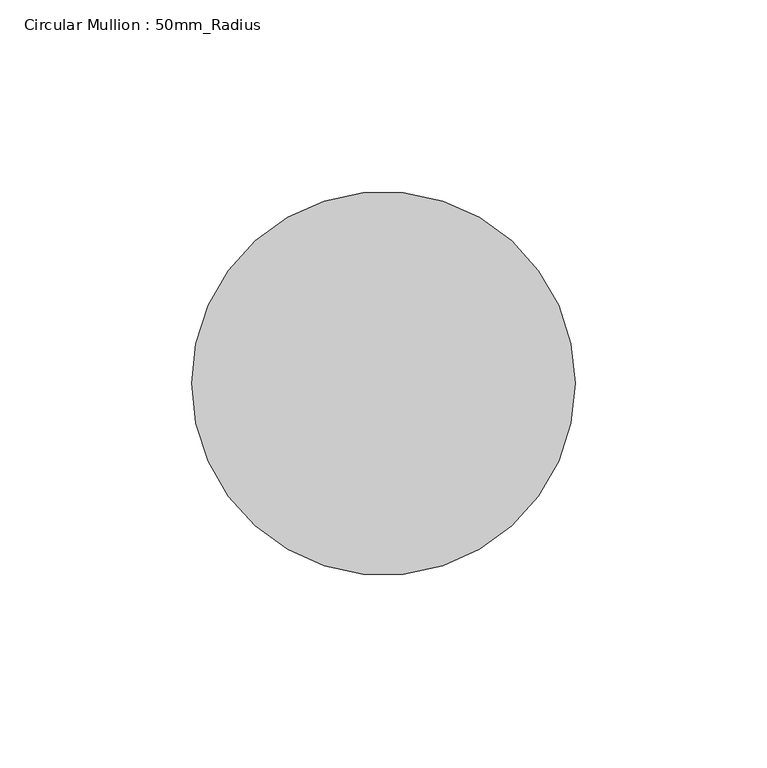
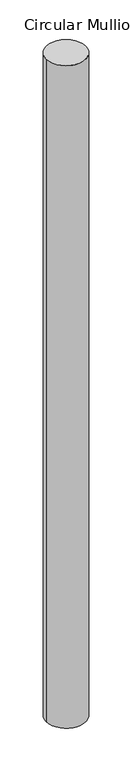
"""IFC4 building model written with IfcOpenShell, lengths in millimetres: member geometry, Circular Mullion : 50mm_Radius."""

from ifc_helpers import new_model, si_unit, point, frame, origin, origin_2d, place, context, project, spatial, circle_curve, trimmed, segment, composite_curve, outline, extrude, source, transform, mapped, element, save


def circular_mullion_50mm_radius_686eca1b(model_context):
    return source(origin(), model_context, "Body", "SweptSolid", [
        extrude(outline(composite_curve([segment(trimmed(circle_curve(origin_2d(), 50.0), [point((50.0, 0.0))], [point((-50.0, 0.0))], False, "CARTESIAN"), True, "CONTINUOUS"), segment(trimmed(circle_curve(origin_2d(), 50.0), [point((-50.0, 0.0))], [point((50.0, 0.0))], False, "CARTESIAN"), True, "CONTINUOUS")], self_intersect=False)), frame((0.0, 0.0, -1780.0), z_axis=(0.0, 0.0, 1.0), x_axis=(1.0, 0.0, 0.0)), (0.0, 0.0, 1.0), 1780.0),
    ])


if __name__ == "__main__":
    model = new_model("IFC4")
    model_context = context("Model", 3, world=origin())
    ifc_project = project(units=[si_unit("LENGTHUNIT", "METRE", prefix="MILLI")], contexts=[model_context])
    site = spatial("IfcSite", under=ifc_project)
    building = spatial("IfcBuilding", under=site)
    placement = place(None, origin())
    circular_mullion_50mm_radius_shape = circular_mullion_50mm_radius_686eca1b(model_context)
    element("IfcMember", 1, ObjectType="Circular Mullion : 50mm_Radius", at=placement, inside=building, context=model_context, shape_type="MappedRepresentation", body=[
        mapped(circular_mullion_50mm_radius_shape, transform((0.0, 0.0, 0.0), x_axis=(1.0, 0.0, 0.0), y_axis=(0.0, 1.0, 0.0), z_axis=(0.0, 0.0, 1.0))),
    ])
    save(model, "model.ifc")

# Revit data of these elements
# Type "Circular Mullion : 50mm_Radius"
#   Keynote = "H11"
#   built-in parameter 1007350 = 0.164042 (stored number, unit not read)
# Element 1 (IfcMember, "Circular Mullion : 50mm_Radius")
#   Materials on its faces: "Aluminium"
# Materials
#   "Aluminium": class "Metal", colour RGB 247 247 247, transparency 0, Description = "Aluminium 6061", Cost = 0
